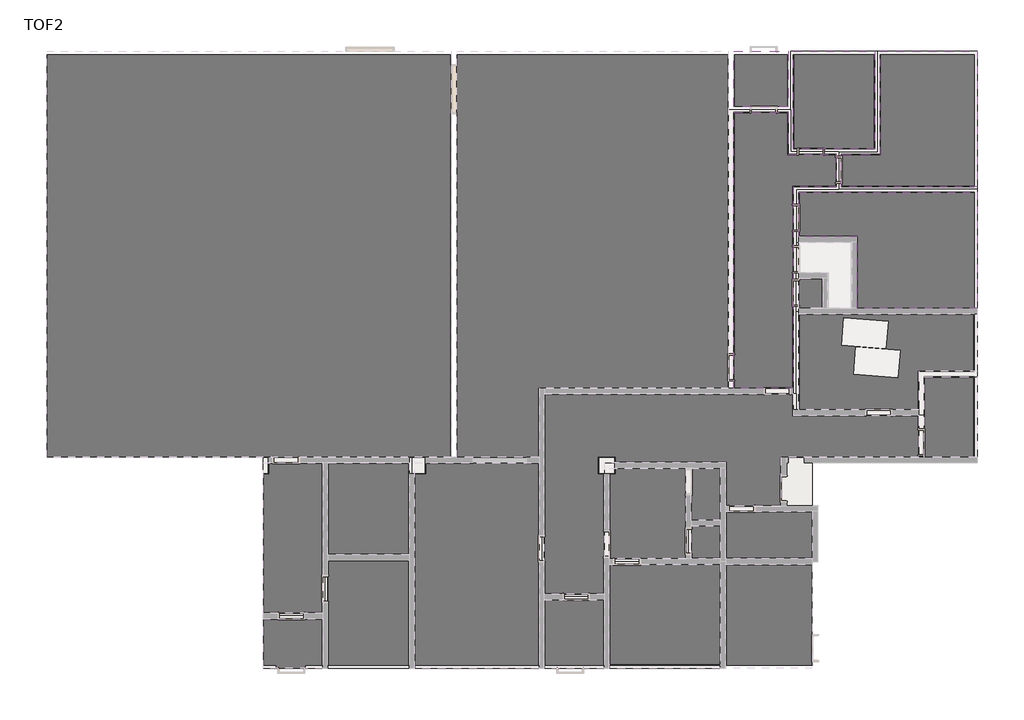
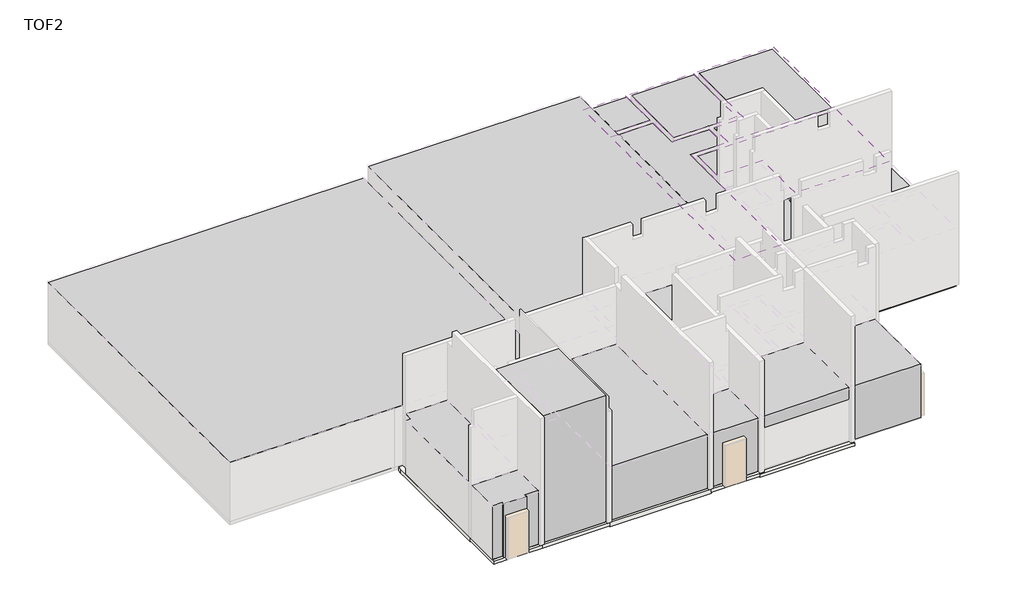
# One storey, part 5 of 5: 24 slabs, 23 proxies, 5 coverings.
# Revit data of these elements (continued)
# Room at (30057.5, 6598.271) mm, phase "New Construction", upper level "TOC", upper offset 2000 mm, lower offset 0 mm (continued)
#   Floor Finish Style No = F34A
#   Skirt Finish Style No = B35
#   Wall Finish Style No = W01B
#   Ceiling Finish Style No = C95A
# Room at (27362.5, 1628.771) mm, phase "New Construction", upper level "TOC", upper offset 2000 mm, lower offset 0 mm
#   Comments = ""
#   Number = "117"
#   Name = "AIR LOCK"
#   H_Floor Finish Style Name = "Vinyl Tile"
#   H_Floor Base Material = "Concrete Slab / Steel Trowel Finish"
#   H_Wall-Base Material-1 = "Masonry Wall"
#   H_Skirt Finish Style Name = "Coved Vinyl Tile"
#   H_Wall-Base Material-2 = ""
#   H_Wall-Base Material-3 = "Plastering"
#   H_Floor-Base Material-1 = "Concrete Slab"
#   H_Floor-Base Material-2 = "Steel Trowel Finish"
#   H_Floor-Base Material-3 = ""
#   H_Floor-Base Material-4 = ""
#   H_Floor-Base Material-5 = "Vinyl Tile"
#   H_Floor Finish-1 = "Vinyl Tile"
#   H_Floor Finish-2 = ""
#   H_Floor Finish Remark = ""
#   H_Skirt Base Material = "Same as Wall"
#   H_Skirt-Base Material-1 = ""
#   H_Skirt-Base Material-2 = ""
#   H_Skirt-Base Material-3 = ""
#   H_Skirt-Base Material-4 = ""
#   H_Skirt-Base Material-5 = ""
#   H_Skirt Finish-1 = "Vinyl Tile"
#   H_Skirt Finish-2 = ""
#   H_Skirt Finish Remark = "Vinyl Tile = PVC Tile (polyvinyl chloride)"
#   H_Wall Finish Style Name = "Acrylic Emulsion Paint"
#   H_Wall Base Material = "Masonry Wall / Cement Plaster"
#   H_Wall-Base Material-4 = ""
#   H_Wall-Base Material-5 = ""
#   H_Wall Finish-1 = "Acrylic Emulsion Paint"
#   H_Wall Finish-2 = ""
#   H_Wall Finish Remark = "T13 Plaster"
#   H_Ceiling Finish Style Name = "Suspended Acoustic Tiled Ceiling (M-Bar)"
#   H_Ceiling Base Material = "Concrete Slab / Fair Faced Concrete"
#   H_Ceiling-Base Material-1 = "(Concrete Slab)"
#   H_Ceiling-Base Material-2 = "(Fair Faced Concrete)"
#   H_Ceiling-Base Material-3 = ""
#   H_Ceiling-Base Material-4 = ""
#   H_Ceiling-Base Material-5 = "Acoustic Tiled Ceiling System (M-Bar)"
#   H_Ceiling Finish-1 = "Acoustic Tiled Ceiling System (M-Bar)"
#   H_Ceiling Finish-2 = ""
#   H_Ceiling Finish Remark = ""
#   H_Room W = 2100 mm
#   H_Room L = 5500 mm
#   H_Room H or CH = 2600 mm
#   Floor Finish Style No = F34A
#   Skirt Finish Style No = B35
#   Wall Finish Style No = W01B
#   Ceiling Finish Style No = C95A
# Room at (27362.5, 5760.771) mm, phase "New Construction", upper level "TOC", upper offset 2000 mm, lower offset 0 mm
#   Comments = ""
#   Number = "116"
#   Name = "CORRIDOR"
#   H_Floor Finish Style Name = "Vinyl Tile"
#   H_Floor Base Material = "Concrete Slab / Steel Trowel Finish"
#   H_Wall-Base Material-1 = "Masonry Wall"
#   H_Skirt Finish Style Name = "Coved Vinyl Tile"
#   H_Wall-Base Material-2 = ""
#   H_Wall-Base Material-3 = "Plastering"
#   H_Floor-Base Material-1 = "Concrete Slab"
#   H_Floor-Base Material-2 = "Steel Trowel Finish"
#   H_Floor-Base Material-3 = ""
#   H_Floor-Base Material-4 = ""
#   H_Floor-Base Material-5 = "Vinyl Tile"
#   H_Floor Finish-1 = "Vinyl Tile"
#   H_Floor Finish-2 = ""
#   H_Floor Finish Remark = ""
#   H_Skirt Base Material = "Same as Wall"
#   H_Skirt-Base Material-1 = ""
#   H_Skirt-Base Material-2 = ""
#   H_Skirt-Base Material-3 = ""
#   H_Skirt-Base Material-4 = ""
#   H_Skirt-Base Material-5 = ""
#   H_Skirt Finish-1 = "Vinyl Tile"
#   H_Skirt Finish-2 = ""
#   H_Skirt Finish Remark = "Vinyl Tile = PVC Tile (polyvinyl chloride)"
#   H_Wall Finish Style Name = "Acrylic Emulsion Paint"
#   H_Wall Base Material = "Masonry Wall / Cement Plaster"
#   H_Wall-Base Material-4 = ""
#   H_Wall-Base Material-5 = ""
#   H_Wall Finish-1 = "Acrylic Emulsion Paint"
#   H_Wall Finish-2 = ""
#   H_Wall Finish Remark = "T13 Plaster"
#   H_Ceiling Finish Style Name = "Suspended Acoustic Tiled Ceiling (M-Bar)"
#   H_Ceiling Base Material = "Concrete Slab / Fair Faced Concrete"
#   H_Ceiling-Base Material-1 = "(Concrete Slab)"
#   H_Ceiling-Base Material-2 = "(Fair Faced Concrete)"
#   H_Ceiling-Base Material-3 = ""
#   H_Ceiling-Base Material-4 = ""
#   H_Ceiling-Base Material-5 = "Acoustic Tiled Ceiling System (M-Bar)"
#   H_Ceiling Finish-1 = "Acoustic Tiled Ceiling System (M-Bar)"
#   H_Ceiling Finish-2 = ""
#   H_Ceiling Finish Remark = ""
#   H_Room W = 13800 mm
#   H_Room L = 7300 mm
#   H_Room H or CH = 2600 mm
#   Floor Finish Style No = F34A
#   Skirt Finish Style No = B35
#   Wall Finish Style No = W01B
#   Ceiling Finish Style No = C95A
# Room at (43870, 7604.869) mm, phase "New Construction", upper level "TOC", upper offset 2000 mm, lower offset 0 mm
#   Comments = ""
#   Number = "120"
#   Name = "CORRIDOR"
#   H_Floor Finish Style Name = "Vinyl Tile"
#   H_Floor Base Material = "Concrete Slab / Steel Trowel Finish"
#   H_Wall-Base Material-1 = "Masonry Wall"
#   H_Skirt Finish Style Name = "Coved Vinyl Tile"
#   H_Wall-Base Material-2 = ""
#   H_Wall-Base Material-3 = "Plastering"
#   H_Floor-Base Material-1 = "Concrete Slab"
#   H_Floor-Base Material-2 = "Steel Trowel Finish"
#   H_Floor-Base Material-3 = ""
#   H_Floor-Base Material-4 = ""
#   H_Floor-Base Material-5 = "Vinyl Tile"
#   H_Floor Finish-1 = "Vinyl Tile"
#   H_Floor Finish-2 = ""
#   H_Floor Finish Remark = ""
#   H_Skirt Base Material = "Same as Wall"
#   H_Skirt-Base Material-1 = ""
#   H_Skirt-Base Material-2 = ""
#   H_Skirt-Base Material-3 = ""
#   H_Skirt-Base Material-4 = ""
#   H_Skirt-Base Material-5 = ""
#   H_Skirt Finish-1 = "Vinyl Tile"
#   H_Skirt Finish-2 = ""
#   H_Skirt Finish Remark = "Vinyl Tile = PVC Tile (polyvinyl chloride)"
#   H_Wall Finish Style Name = "Acrylic Emulsion Paint"
#   H_Wall Base Material = "Masonry Wall / Cement Plaster"
#   H_Wall-Base Material-4 = ""
#   H_Wall-Base Material-5 = ""
#   H_Wall Finish-1 = "Acrylic Emulsion Paint"
#   H_Wall Finish-2 = ""
#   H_Wall Finish Remark = "T13 Plaster"
#   H_Ceiling Finish Style Name = "Suspended Acoustic Tiled Ceiling (M-Bar)"
#   H_Ceiling Base Material = "Concrete Slab / Fair Faced Concrete"
#   H_Ceiling-Base Material-1 = "(Concrete Slab)"
#   H_Ceiling-Base Material-2 = "(Fair Faced Concrete)"
#   H_Ceiling-Base Material-3 = ""
#   H_Ceiling-Base Material-4 = ""
#   H_Ceiling-Base Material-5 = "Acoustic Tiled Ceiling System (M-Bar)"
#   H_Ceiling Finish-1 = "Acoustic Tiled Ceiling System (M-Bar)"
#   H_Ceiling Finish-2 = ""
#   H_Ceiling Finish Remark = ""
#   H_Room W = 2100 mm
#   H_Room L = 2400 mm
#   H_Room H or CH = 2600 mm
#   Floor Finish Style No = F34A
#   Skirt Finish Style No = B35
#   Wall Finish Style No = W01B
#   Ceiling Finish Style No = C95A
# Room at (37870, 1977.173) mm, phase "New Construction", upper level "TOC", upper offset 2000 mm, lower offset 0 mm
#   Comments = ""
#   Number = "119"
#   Name = "AIR LOCK"
#   H_Floor Finish Style Name = "Vinyl Tile"
#   H_Floor Base Material = "Concrete Slab / Steel Trowel Finish"
#   H_Wall-Base Material-1 = "Masonry Wall"
#   H_Skirt Finish Style Name = "Coved Vinyl Tile"
#   H_Wall-Base Material-2 = ""
#   H_Wall-Base Material-3 = "Plastering"
#   H_Floor-Base Material-1 = "Concrete Slab"
#   H_Floor-Base Material-2 = "Steel Trowel Finish"
#   H_Floor-Base Material-3 = ""
#   H_Floor-Base Material-4 = ""
#   H_Floor-Base Material-5 = "Vinyl Tile"
#   H_Floor Finish-1 = "Vinyl Tile"
#   H_Floor Finish-2 = ""
#   H_Floor Finish Remark = ""
#   H_Skirt Base Material = "Same as Wall"
#   H_Skirt-Base Material-1 = ""
#   H_Skirt-Base Material-2 = ""
#   H_Skirt-Base Material-3 = ""
#   H_Skirt-Base Material-4 = ""
#   H_Skirt-Base Material-5 = ""
#   H_Skirt Finish-1 = "Vinyl Tile"
#   H_Skirt Finish-2 = ""
#   H_Skirt Finish Remark = "Vinyl Tile = PVC Tile (polyvinyl chloride)"
#   H_Wall Finish Style Name = "Acrylic Emulsion Paint"
#   H_Wall Base Material = "Masonry Wall / Cement Plaster"
#   H_Wall-Base Material-4 = ""
#   H_Wall-Base Material-5 = ""
#   H_Wall Finish-1 = "Acrylic Emulsion Paint"
#   H_Wall Finish-2 = ""
#   H_Wall Finish Remark = "T13 Plaster"
#   H_Ceiling Finish Style Name = "Suspended Acoustic Tiled Ceiling (M-Bar)"
#   H_Ceiling Base Material = "Concrete Slab / Fair Faced Concrete"
#   H_Ceiling-Base Material-1 = "(Concrete Slab)"
#   H_Ceiling-Base Material-2 = "(Fair Faced Concrete)"
#   H_Ceiling-Base Material-3 = ""
#   H_Ceiling-Base Material-4 = ""
#   H_Ceiling-Base Material-5 = "Acoustic Tiled Ceiling System (M-Bar)"
#   H_Ceiling Finish-1 = "Acoustic Tiled Ceiling System (M-Bar)"
#   H_Ceiling Finish-2 = ""
#   H_Ceiling Finish Remark = ""
#   H_Room W = 2400 mm
#   H_Room L = 2500 mm
#   H_Room H or CH = 2700 mm
#   Floor Finish Style No = F34A
#   Skirt Finish Style No = B35
#   Wall Finish Style No = W01B
#   Ceiling Finish Style No = C95A
